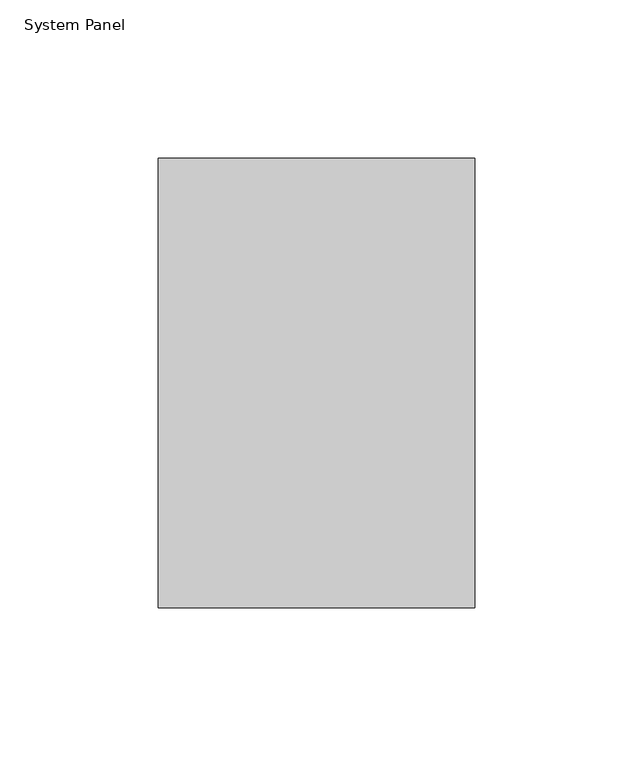
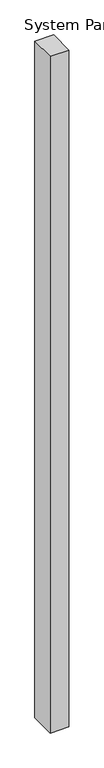
"""IFC4 building model written with IfcOpenShell, lengths in millimetres: plate geometry, System Panel : NLRS_21_CWP_hsb-vulling minerale wol 142 _gen_rsf."""

from ifc_helpers import new_model, si_unit, origin, origin_with_axes, place, context, project, spatial, polyline, outline, extrude, source, transform, mapped, element, save


def system_panel_45496c6a(model_context):
    return source(origin(), model_context, "Body", "SweptSolid", [
        extrude(outline(polyline([(49.9999998, -71.0), (-49.9999998, -71.0), (-49.9999998, 71.0), (49.9999998, 71.0), (49.9999998, -71.0)])), origin_with_axes(), (0.0, 0.0, 1.0), 3849.0),
    ])


if __name__ == "__main__":
    model = new_model("IFC4")
    model_context = context("Model", 3, world=origin())
    ifc_project = project(units=[si_unit("LENGTHUNIT", "METRE", prefix="MILLI")], contexts=[model_context])
    site = spatial("IfcSite", under=ifc_project)
    building = spatial("IfcBuilding", under=site)
    placement = place(None, origin())
    system_panel_shape = system_panel_45496c6a(model_context)
    element("IfcPlate", 1, ObjectType="System Panel : NLRS_21_CWP_hsb-vulling minerale wol 142 _gen_rsf", at=placement, inside=building, context=model_context, shape_type="MappedRepresentation", body=[
        mapped(system_panel_shape, transform((0.0, 0.0, 0.0), x_axis=(1.0, 0.0, 0.0), y_axis=(0.0, 1.0, 0.0), z_axis=(0.0, 0.0, 1.0))),
    ])
    save(model, "model.ifc")

# Revit data of these elements
# Type "System Panel : NLRS_21_CWP_hsb-vulling minerale wol 142 _gen_rsf"
#   Export Type to IFC As = "IfcWall"
#   Type IfcGUID = "07M7mRoiH1CR8m_RSKIwpC"
#   Assembly Code = "21.23"
# Element 1 (IfcPlate, "System Panel : NLRS_21_CWP_hsb-vulling minerale wol 142 _gen_rsf")
#   Materials on its faces: "NLRS_m1_isolatie minerale wol_gen_rsf"
# Materials
#   "NLRS_m1_isolatie minerale wol_gen_rsf": class "M - Anorganische materialen", colour RGB 200 200 140, transparency 0, Keynote = "m1", Manufacturer = "Revit Standards Foundation", URL = "www.revitstandards.org", Description = "isolatie minerale wol", Cost = 0
